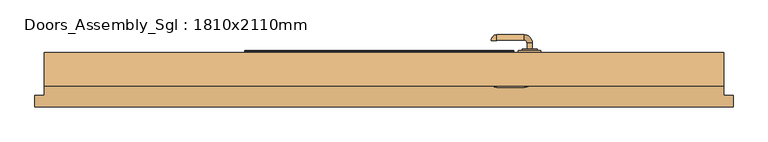
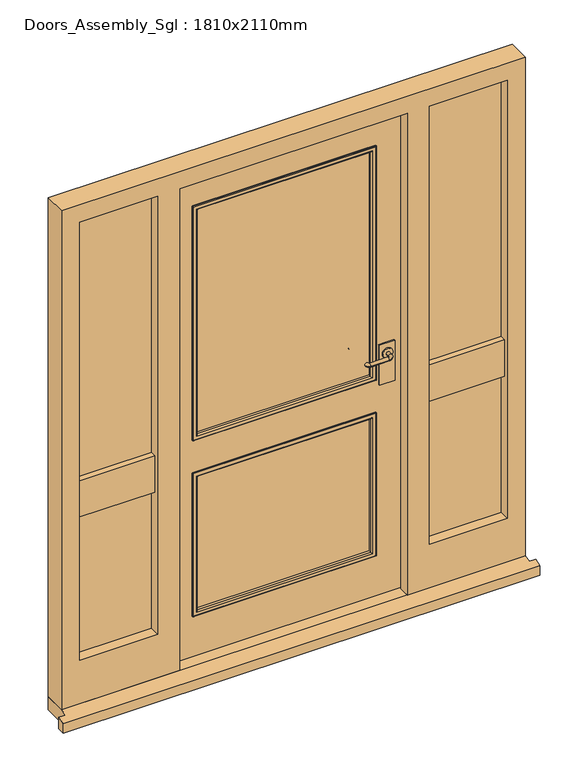
"""IFC4 building model written with IfcOpenShell, lengths in millimetres: door geometry, Doors_Assembly_Sgl : 1810x2110mm."""

from ifc_helpers import new_model, si_unit, point, frame, frame_2d, origin, place, context, project, spatial, polyline, circle_curve, ellipse_curve, trimmed, segment, composite_curve, outline, extrude, faceted_brep, source, transform, mapped, element, save
from ifc_brep_helpers import plane_surface, cylinder_surface, revolved_surface, advanced_brep


def doors_assembly_sgl_1810x2110mm_cdd653b2(model_context):
    return source(origin(), model_context, "Body", "SolidModel", [
        extrude(outline(composite_curve([segment(trimmed(circle_curve(frame_2d((1050.0, 680.0)), 20.0), [point((1050.0, 700.0))], [point((1050.0, 660.0))], False, "CARTESIAN"), True, "CONTINUOUS"), segment(trimmed(circle_curve(frame_2d((1050.0, 680.0)), 20.0), [point((1050.0, 660.0))], [point((1050.0, 700.0))], False, "CARTESIAN"), True, "CONTINUOUS")], self_intersect=False)), frame((0.0, -42.25, 0.0), z_axis=(0.0, 1.0, 0.0), x_axis=(0.0, 0.0, 1.0)), (0.0, 0.0, 1.0), 4.5929895),
        advanced_brep(
        [(673.0, -37.6570105, 1050.0), (687.0, -37.6570105, 1050.0), (687.0, -22.25, 1050.0), (673.0, -22.25, 1050.0), (665.0, -0.25, 1050.0), (665.0, -14.25, 1050.0), (593.0, -0.25, 1050.0), (593.0, -14.25, 1050.0), (592.0, -15.25, 1050.0), (578.0, -15.25, 1050.0)],
        [
            (0, 1, circle_curve(frame((680.0, -37.6570105, 1050.0), z_axis=(0.0, -1.0, 0.0), x_axis=(1.0, 0.0, 0.0)), 7.0)),
            (1, 0, circle_curve(frame((680.0, -37.6570105, 1050.0), z_axis=(0.0, -1.0, 0.0), x_axis=(1.0, 0.0, 0.0)), 7.0)),
            (1, 2),
            (2, 3, circle_curve(frame((680.0, -22.25, 1050.0), z_axis=(0.0, -1.0, 0.0), x_axis=(1.0, 0.0, 0.0)), 7.0)),
            (3, 0),
            (3, 2, circle_curve(frame((680.0, -22.25, 1050.0), z_axis=(0.0, -1.0, 0.0), x_axis=(1.0, 0.0, 0.0)), 7.0)),
            (4, 5, circle_curve(frame((665.0, -7.25, 1050.0), z_axis=(1.0, 0.0, 0.0), x_axis=(0.0, 1.0, 0.0)), 7.0)),
            (5, 3, circle_curve(frame((665.0, -22.25, 1050.0), z_axis=(0.0, 0.0, -1.0), x_axis=(1.0, 0.0, 0.0)), 8.0)),
            (2, 4, circle_curve(frame((665.0, -22.25, 1050.0), z_axis=(0.0, 0.0, 1.0), x_axis=(1.0, 0.0, 0.0)), 22.0)),
            (5, 4, circle_curve(frame((665.0, -7.25, 1050.0), z_axis=(1.0, 0.0, 0.0), x_axis=(0.0, 1.0, 0.0)), 7.0)),
            (4, 6),
            (6, 7, circle_curve(frame((593.0, -7.25, 1050.0), z_axis=(1.0, 0.0, 0.0), x_axis=(0.0, 1.0, 0.0)), 7.0)),
            (7, 5),
            (7, 6, circle_curve(frame((593.0, -7.25, 1050.0), z_axis=(1.0, 0.0, 0.0), x_axis=(0.0, 1.0, 0.0)), 7.0)),
            (8, 9, circle_curve(frame((585.0, -15.25, 1050.0), z_axis=(0.0, -1.0, 0.0), x_axis=(-1.0, 0.0, 0.0)), 7.0)),
            (9, 8, circle_curve(frame((585.0, -15.25, 1050.0), z_axis=(0.0, -1.0, 0.0), x_axis=(-1.0, 0.0, 0.0)), 7.0)),
            (8, 7, circle_curve(frame((593.0, -15.25, 1050.0), z_axis=(0.0, 0.0, -1.0), x_axis=(0.0, 1.0, 0.0)), 1.0)),
            (6, 9, circle_curve(frame((593.0, -15.25, 1050.0), z_axis=(0.0, 0.0, 1.0), x_axis=(0.0, 1.0, 0.0)), 15.0)),
        ],
        [
            plane_surface(frame((680.0, -37.6570105, 1050.0), z_axis=(0.0, -1.0, 0.0), x_axis=(0.0, 0.0, 1.0))),
            cylinder_surface(frame((680.0, -37.6570105, 1050.0), z_axis=(0.0, -1.0, 0.0), x_axis=(1.0, 0.0, 0.0)), 7.0),
            revolved_surface(trimmed(ellipse_curve(frame((680.0, -22.25, 1050.0), z_axis=(0.0, 1.0, 0.0), x_axis=(1.0, 0.0, 0.0)), 7.0, 7.0), [point((673.0, -22.25, 1050.0))], [point((687.0, -22.25, 1050.0))], True, "CARTESIAN"), (665.0, -22.25, 1050.0), (0.0, 0.0, -1.0)),
            revolved_surface(trimmed(ellipse_curve(frame((680.0, -22.25, 1050.0), z_axis=(0.0, 1.0, 0.0), x_axis=(1.0, 0.0, 0.0)), 7.0, 7.0), [point((687.0, -22.25, 1050.0))], [point((673.0, -22.25, 1050.0))], True, "CARTESIAN"), (665.0, -22.25, 1050.0), (0.0, 0.0, -1.0)),
            cylinder_surface(frame((665.0, -7.25, 1050.0), z_axis=(1.0, 0.0, 0.0), x_axis=(0.0, 1.0, 0.0)), 7.0),
            plane_surface(frame((585.0, -15.25, 1050.0), z_axis=(0.0, -1.0, 0.0), x_axis=(0.0, 0.0, 1.0))),
            revolved_surface(trimmed(ellipse_curve(frame((593.0, -7.25, 1050.0), z_axis=(-1.0, 0.0, 0.0), x_axis=(0.0, 1.0, 0.0)), 7.0, 7.0), [point((593.0, -14.25, 1050.0))], [point((593.0, -0.25, 1050.0))], True, "CARTESIAN"), (593.0, -15.25, 1050.0), (0.0, 0.0, -1.0)),
            revolved_surface(trimmed(ellipse_curve(frame((593.0, -7.25, 1050.0), z_axis=(-1.0, 0.0, 0.0), x_axis=(0.0, 1.0, 0.0)), 7.0, 7.0), [point((593.0, -0.25, 1050.0))], [point((593.0, -14.25, 1050.0))], True, "CARTESIAN"), (593.0, -15.25, 1050.0), (0.0, 0.0, -1.0)),
        ],
        [
            (0, [[1, 2]]),
            (1, [[3, 4, 5, -2]]),
            (1, [[-5, 6, -3, -1]]),
            (2, [[7, 8, -4, 9]]),
            (3, [[10, -9, -6, -8]]),
            (4, [[11, 12, 13, -7]]),
            (4, [[-13, 14, -11, -10]]),
            (5, [[15, 16]]),
            (6, [[-15, 17, -12, 18]]),
            (7, [[-16, -18, -14, -17]]),
        ],
    ),
        extrude(outline(polyline([(650.0, -48.25), (650.0, -42.25), (710.0, -42.25), (710.0, -48.25), (650.0, -48.25)])), frame((0.0, 0.0, 925.0), z_axis=(0.0, 0.0, 1.0), x_axis=(1.0, 0.0, 0.0)), (0.0, 0.0, 1.0), 165.0),
        extrude(outline(composite_curve([segment(trimmed(circle_curve(frame_2d((1050.0, 680.0)), 20.0), [point((1050.0, 700.0))], [point((1050.0, 660.0))], False, "CARTESIAN"), True, "CONTINUOUS"), segment(trimmed(circle_curve(frame_2d((1050.0, 680.0)), 20.0), [point((1050.0, 660.0))], [point((1050.0, 700.0))], False, "CARTESIAN"), True, "CONTINUOUS")], self_intersect=False)), frame((0.0, -102.8429895, 0.0), z_axis=(0.0, 1.0, 0.0), x_axis=(0.0, 0.0, 1.0)), (0.0, 0.0, 1.0), 4.5929895),
        advanced_brep(
        [(673.0, -102.8429895, 1050.0), (687.0, -102.8429895, 1050.0), (673.0, -118.25, 1050.0), (687.0, -118.25, 1050.0), (665.0, -140.25, 1050.0), (665.0, -126.25, 1050.0), (593.0, -126.25, 1050.0), (593.0, -140.25, 1050.0), (592.0, -125.25, 1050.0), (578.0, -125.25, 1050.0)],
        [
            (0, 1, circle_curve(frame((680.0, -102.8429895, 1050.0), z_axis=(0.0, 1.0, 0.0), x_axis=(1.0, 0.0, 0.0)), 7.0)),
            (1, 0, circle_curve(frame((680.0, -102.8429895, 1050.0), z_axis=(0.0, 1.0, 0.0), x_axis=(1.0, 0.0, 0.0)), 7.0)),
            (0, 2),
            (2, 3, circle_curve(frame((680.0, -118.25, 1050.0), z_axis=(0.0, 1.0, 0.0), x_axis=(1.0, 0.0, 0.0)), 7.0)),
            (3, 1),
            (3, 2, circle_curve(frame((680.0, -118.25, 1050.0), z_axis=(0.0, 1.0, 0.0), x_axis=(1.0, 0.0, 0.0)), 7.0)),
            (4, 3, circle_curve(frame((665.0, -118.25, 1050.0), z_axis=(0.0, 0.0, 1.0), x_axis=(1.0, 0.0, 0.0)), 22.0)),
            (2, 5, circle_curve(frame((665.0, -118.25, 1050.0), z_axis=(0.0, 0.0, -1.0), x_axis=(1.0, 0.0, 0.0)), 8.0)),
            (5, 4, circle_curve(frame((665.0, -133.25, 1050.0), z_axis=(1.0, 0.0, 0.0), x_axis=(0.0, -1.0, 0.0)), 7.0)),
            (4, 5, circle_curve(frame((665.0, -133.25, 1050.0), z_axis=(1.0, 0.0, 0.0), x_axis=(0.0, -1.0, 0.0)), 7.0)),
            (5, 6),
            (6, 7, circle_curve(frame((593.0, -133.25, 1050.0), z_axis=(1.0, 0.0, 0.0), x_axis=(0.0, -1.0, 0.0)), 7.0)),
            (7, 4),
            (7, 6, circle_curve(frame((593.0, -133.25, 1050.0), z_axis=(1.0, 0.0, 0.0), x_axis=(0.0, -1.0, 0.0)), 7.0)),
            (8, 9, circle_curve(frame((585.0, -125.25, 1050.0), z_axis=(0.0, 1.0, 0.0), x_axis=(-1.0, 0.0, 0.0)), 7.0)),
            (9, 8, circle_curve(frame((585.0, -125.25, 1050.0), z_axis=(0.0, 1.0, 0.0), x_axis=(-1.0, 0.0, 0.0)), 7.0)),
            (9, 7, circle_curve(frame((593.0, -125.25, 1050.0), z_axis=(0.0, 0.0, 1.0), x_axis=(0.0, -1.0, 0.0)), 15.0)),
            (6, 8, circle_curve(frame((593.0, -125.25, 1050.0), z_axis=(0.0, 0.0, -1.0), x_axis=(0.0, -1.0, 0.0)), 1.0)),
        ],
        [
            plane_surface(frame((680.0, -102.8429895, 1050.0), z_axis=(0.0, 1.0, 0.0), x_axis=(0.0, 0.0, 1.0))),
            cylinder_surface(frame((680.0, -102.8429895, 1050.0), z_axis=(0.0, 1.0, 0.0), x_axis=(1.0, 0.0, 0.0)), 7.0),
            revolved_surface(trimmed(ellipse_curve(frame((680.0, -118.25, 1050.0), z_axis=(0.0, 1.0, 0.0), x_axis=(1.0, 0.0, 0.0)), 7.0, 7.0), [point((673.0, -118.25, 1050.0))], [point((687.0, -118.25, 1050.0))], True, "CARTESIAN"), (665.0, -118.25, 1050.0), (0.0, 0.0, -1.0)),
            revolved_surface(trimmed(ellipse_curve(frame((680.0, -118.25, 1050.0), z_axis=(0.0, 1.0, 0.0), x_axis=(1.0, 0.0, 0.0)), 7.0, 7.0), [point((687.0, -118.25, 1050.0))], [point((673.0, -118.25, 1050.0))], True, "CARTESIAN"), (665.0, -118.25, 1050.0), (0.0, 0.0, -1.0)),
            cylinder_surface(frame((665.0, -133.25, 1050.0), z_axis=(1.0, 0.0, 0.0), x_axis=(0.0, -1.0, 0.0)), 7.0),
            plane_surface(frame((585.0, -125.25, 1050.0), z_axis=(0.0, 1.0, 0.0), x_axis=(0.0, 0.0, 1.0))),
            revolved_surface(trimmed(ellipse_curve(frame((593.0, -133.25, 1050.0), z_axis=(1.0, 0.0, 0.0), x_axis=(0.0, -1.0, 0.0)), 7.0, 7.0), [point((593.0, -126.25, 1050.0))], [point((593.0, -140.25, 1050.0))], True, "CARTESIAN"), (593.0, -125.25, 1050.0), (0.0, 0.0, -1.0)),
            revolved_surface(trimmed(ellipse_curve(frame((593.0, -133.25, 1050.0), z_axis=(1.0, 0.0, 0.0), x_axis=(0.0, -1.0, 0.0)), 7.0, 7.0), [point((593.0, -140.25, 1050.0))], [point((593.0, -126.25, 1050.0))], True, "CARTESIAN"), (593.0, -125.25, 1050.0), (0.0, 0.0, -1.0)),
        ],
        [
            (0, [[1, 2]]),
            (1, [[-1, 3, 4, 5]]),
            (1, [[-2, -5, 6, -3]]),
            (2, [[7, -4, 8, 9]]),
            (3, [[-8, -6, -7, 10]]),
            (4, [[-9, 11, 12, 13]]),
            (4, [[-10, -13, 14, -11]]),
            (5, [[15, 16]]),
            (6, [[17, -12, 18, -16]]),
            (7, [[-18, -14, -17, -15]]),
        ],
    ),
        extrude(outline(polyline([(650.0, -92.25), (710.0, -92.25), (710.0, -98.25), (650.0, -98.25), (650.0, -92.25)])), frame((0.0, 0.0, 925.0), z_axis=(0.0, 0.0, 1.0), x_axis=(1.0, 0.0, 0.0)), (0.0, 0.0, 1.0), 165.0),
        extrude(outline(polyline([(1148.5, -71.25), (1148.5, -95.25), (800.0, -95.25), (800.0, -71.25), (1148.5, -71.25)])), frame((0.0, 0.0, 218.5), z_axis=(0.0, 0.0, 1.0), x_axis=(1.0, 0.0, 0.0)), (0.0, 0.0, 1.0), 605.0),
        extrude(outline(polyline([(1148.5, -71.25), (1148.5, -95.25), (800.0, -95.25), (800.0, -71.25), (1148.5, -71.25)])), frame((0.0, 0.0, 943.5), z_axis=(0.0, 0.0, 1.0), x_axis=(1.0, 0.0, 0.0)), (0.0, 0.0, 1.0), 1118.0),
        extrude(outline(polyline([(-216.0, -71.25), (-216.0, -95.25), (-564.5, -95.25), (-564.5, -71.25), (-216.0, -71.25)])), frame((0.0, 0.0, 218.5), z_axis=(0.0, 0.0, 1.0), x_axis=(1.0, 0.0, 0.0)), (0.0, 0.0, 1.0), 605.0),
        extrude(outline(polyline([(-216.0, -71.25), (-216.0, -95.25), (-564.5, -95.25), (-564.5, -71.25), (-216.0, -71.25)])), frame((0.0, 0.0, 943.5), z_axis=(0.0, 0.0, 1.0), x_axis=(1.0, 0.0, 0.0)), (0.0, 0.0, 1.0), 1118.0),
        faceted_brep([(1197.0, -137.25, 54.5), (736.0, -137.25, 54.5), (736.0, -95.25, 54.5), (758.0, -95.25, 54.5), (758.0, -48.25, 54.5), (1197.0, -48.25, 54.5), (1197.0, -48.25, 2110.0), (1197.0, -137.25, 2110.0), (758.0, -48.25, 2061.5), (-174.0, -48.25, 2061.5), (-174.0, -48.25, 54.5), (-613.0, -48.25, 54.5), (-613.0, -48.25, 2110.0), (1126.5, -48.25, 958.5), (1126.5, -48.25, 2039.5), (822.0, -48.25, 2039.5), (822.0, -48.25, 958.5), (822.0, -48.25, 808.5), (822.0, -48.25, 233.5), (1126.5, -48.25, 233.5), (1126.5, -48.25, 808.5), (-238.0, -48.25, 808.5), (-542.5, -48.25, 808.5), (-542.5, -48.25, 233.5), (-238.0, -48.25, 233.5), (-542.5, -48.25, 2039.5), (-542.5, -48.25, 958.5), (-238.0, -48.25, 958.5), (-238.0, -48.25, 2039.5), (758.0, -95.25, 2061.5), (-174.0, -95.25, 54.5), (-174.0, -95.25, 2061.5), (736.0, -95.25, 2039.5), (-152.0, -95.25, 2039.5), (-152.0, -95.25, 54.5), (-216.0, -95.25, 2061.5), (-216.0, -95.25, 943.5), (-564.5, -95.25, 943.5), (-564.5, -95.25, 2061.5), (-542.5, -95.25, 2039.5), (-542.5, -95.25, 958.5), (-238.0, -95.25, 958.5), (-238.0, -95.25, 2039.5), (1148.5, -95.25, 2061.5), (1148.5, -95.25, 943.5), (800.0, -95.25, 943.5), (800.0, -95.25, 2061.5), (822.0, -95.25, 2039.5), (822.0, -95.25, 958.5), (1126.5, -95.25, 958.5), (1126.5, -95.25, 2039.5), (1148.5, -95.25, 218.5), (800.0, -95.25, 218.5), (800.0, -95.25, 823.5), (1148.5, -95.25, 823.5), (1126.5, -95.25, 808.5), (822.0, -95.25, 808.5), (822.0, -95.25, 233.5), (1126.5, -95.25, 233.5), (-564.5, -95.25, 823.5), (-216.0, -95.25, 823.5), (-216.0, -95.25, 218.5), (-564.5, -95.25, 218.5), (-238.0, -95.25, 808.5), (-542.5, -95.25, 808.5), (-542.5, -95.25, 233.5), (-238.0, -95.25, 233.5), (736.0, -137.25, 2039.5), (-613.0, -137.25, 54.5), (-152.0, -137.25, 54.5), (-152.0, -137.25, 2039.5), (-613.0, -137.25, 2110.0), (-238.0, -137.25, 2039.5), (-238.0, -137.25, 233.5), (-542.5, -137.25, 233.5), (-542.5, -137.25, 2039.5), (1126.5, -137.25, 2039.5), (1126.5, -137.25, 233.5), (822.0, -137.25, 233.5), (822.0, -137.25, 2039.5), (-542.5, -118.25, 808.5), (-542.5, -118.25, 958.5), (-238.0, -118.25, 958.5), (-238.0, -118.25, 808.5), (822.0, -118.25, 808.5), (822.0, -118.25, 958.5), (1126.5, -118.25, 958.5), (1126.5, -118.25, 808.5), (822.0, -71.25, 958.5), (1126.5, -71.25, 958.5), (822.0, -71.25, 2039.5), (822.0, -71.25, 808.5), (822.0, -71.25, 233.5), (1126.5, -71.25, 2039.5), (1126.5, -71.25, 233.5), (1126.5, -71.25, 808.5), (-238.0, -71.25, 958.5), (-238.0, -71.25, 2039.5), (-238.0, -71.25, 233.5), (-238.0, -71.25, 808.5), (-542.5, -71.25, 233.5), (-542.5, -71.25, 2039.5), (-542.5, -71.25, 958.5), (-542.5, -71.25, 808.5), (1148.5, -71.25, 218.5), (1148.5, -71.25, 823.5), (1148.5, -71.25, 943.5), (1148.5, -71.25, 2061.5), (800.0, -71.25, 823.5), (800.0, -71.25, 218.5), (800.0, -71.25, 2061.5), (800.0, -71.25, 943.5), (-564.5, -71.25, 218.5), (-564.5, -71.25, 823.5), (-564.5, -71.25, 943.5), (-564.5, -71.25, 2061.5), (-216.0, -71.25, 943.5), (-216.0, -71.25, 2061.5), (-216.0, -71.25, 823.5), (-216.0, -71.25, 218.5)], [[[0, 1, 2, 3, 4, 5]], [[5, 6, 7, 0]], [[5, 4, 8, 9, 10, 11, 12, 6], [13, 14, 15, 16], [17, 18, 19, 20], [21, 22, 23, 24], [25, 26, 27, 28]], [[3, 29, 8, 4]], [[30, 31, 29, 3, 2, 32, 33, 34]], [[35, 36, 37, 38], [39, 40, 41, 42]], [[43, 44, 45, 46], [47, 48, 49, 50]], [[51, 52, 53, 54], [55, 56, 57, 58]], [[59, 60, 61, 62], [63, 64, 65, 66]], [[1, 67, 32, 2]], [[68, 69, 70, 67, 1, 0, 7, 71], [72, 73, 74, 75], [76, 77, 78, 79]], [[71, 12, 11, 68]], [[34, 33, 70, 69]], [[11, 10, 30, 34, 69, 68]], [[75, 74, 65, 64, 80, 81, 40, 39]], [[65, 74, 73, 66]], [[42, 41, 82, 83, 63, 66, 73, 72]], [[79, 78, 57, 56, 84, 85, 48, 47]], [[77, 58, 57, 78]], [[50, 49, 86, 87, 55, 58, 77, 76]], [[16, 88, 89, 13]], [[90, 88, 16, 15]], [[17, 91, 92, 18]], [[14, 13, 89, 93]], [[19, 94, 95, 20]], [[20, 95, 91, 17]], [[18, 92, 94, 19]], [[28, 27, 96, 97]], [[24, 98, 99, 21]], [[23, 100, 98, 24]], [[101, 102, 26, 25]], [[22, 103, 100, 23]], [[21, 99, 103, 22]], [[26, 102, 96, 27]], [[10, 9, 31, 30]], [[104, 51, 54, 105]], [[106, 44, 43, 107]], [[104, 105, 108, 109], [94, 92, 91, 95]], [[110, 111, 106, 107], [93, 89, 88, 90]], [[54, 53, 108, 105]], [[109, 52, 51, 104]], [[111, 45, 44, 106]], [[40, 81, 82, 41]], [[112, 113, 59, 62]], [[114, 115, 38, 37]], [[37, 36, 116, 114]], [[36, 35, 117, 116]], [[61, 60, 118, 119]], [[48, 85, 86, 49]], [[108, 53, 52, 109]], [[110, 46, 45, 111]], [[55, 87, 84, 56]], [[63, 83, 80, 64]], [[112, 62, 61, 119]], [[113, 118, 60, 59]], [[85, 84, 87, 86]], [[115, 114, 116, 117], [97, 96, 102, 101]], [[119, 118, 113, 112], [100, 103, 99, 98]], [[81, 80, 83, 82]], [[7, 6, 12, 71]], [[9, 8, 29, 31]], [[38, 115, 117, 35]], [[46, 110, 107, 43]], [[76, 79, 47, 50]], [[33, 32, 67, 70]], [[39, 42, 72, 75]], [[101, 25, 28, 97]], [[14, 93, 90, 15]]]),
        extrude(outline(polyline([(-71.0, -82.25), (-71.0, -58.25), (630.0, -58.25), (630.0, -82.25), (-71.0, -82.25)])), frame((0.0, 0.0, 958.5), z_axis=(0.0, 0.0, 1.0), x_axis=(1.0, 0.0, 0.0)), (0.0, 0.0, 1.0), 950.0),
        extrude(outline(polyline([(-71.0, -82.25), (-71.0, -58.25), (630.0, -58.25), (630.0, -82.25), (-71.0, -82.25)])), frame((0.0, 0.0, 233.5), z_axis=(0.0, 0.0, 1.0), x_axis=(1.0, 0.0, 0.0)), (0.0, 0.0, 1.0), 575.0),
        faceted_brep([(1222.0, -192.25, 0.0), (1222.0, -162.25, 0.0), (1222.0, -162.25, 47.2703282), (1222.0, -192.25, 38.5947221), (-638.0, -192.25, 38.5947221), (-638.0, -162.25, 47.2703282), (-638.0, -162.25, 0.0), (-638.0, -192.25, 0.0), (-613.0, -162.25, 0.0), (-613.0, -48.25, 0.0), (1197.0, -48.25, 0.0), (1197.0, -162.25, 0.0), (1197.0, -162.25, 47.2703282), (1197.0, -137.25, 54.5), (-613.0, -137.25, 54.5), (-613.0, -162.25, 47.2703282), (1197.0, -48.25, 54.5), (-613.0, -48.25, 54.5)], [[[0, 1, 2, 3]], [[4, 5, 6, 7]], [[7, 6, 8, 9, 10, 11, 1, 0]], [[3, 4, 7, 0]], [[3, 2, 12, 13, 14, 15, 5, 4]], [[14, 13, 16, 17]], [[17, 16, 10, 9]], [[15, 14, 17, 9, 8]], [[8, 6, 5, 15]], [[11, 10, 16, 13, 12]], [[12, 2, 1, 11]]]),
        extrude(outline(polyline([(58.5, -171.0), (58.5, 755.0), (2058.5, 755.0), (2058.5, -171.0), (58.5, -171.0)]), holes=[polyline([(1908.5, 630.0), (958.5, 630.0), (958.5, -71.0), (1908.5, -71.0), (1908.5, 630.0)]), polyline([(808.5, -71.0), (808.5, 630.0), (233.5, 630.0), (233.5, -71.0), (808.5, -71.0)])]), frame((0.0, -92.25, 0.0), z_axis=(0.0, 1.0, 0.0), x_axis=(0.0, 0.0, 1.0)), (0.0, 0.0, 1.0), 44.0),
        advanced_brep(
        [(630.0, -58.25, 808.5), (630.0, -58.25, 233.5), (630.0, -48.25, 233.5), (630.0, -48.25, 808.5), (618.0, -47.25, 796.5), (618.0, -47.25, 245.5), (618.0, -58.25, 245.5), (618.0, -58.25, 796.5), (623.0, -42.25, 801.5), (623.0, -42.25, 240.5), (638.0, -44.25, 816.5), (638.0, -44.25, 225.5), (636.0, -42.25, 227.5), (636.0, -42.25, 814.5), (638.0, -48.25, 816.5), (638.0, -48.25, 225.5), (-71.0, -58.25, 233.5), (-71.0, -48.25, 233.5), (-59.0, -47.25, 245.5), (-59.0, -58.25, 245.5), (-64.0, -42.25, 240.5), (-79.0, -44.25, 225.5), (-77.0, -42.25, 227.5), (-79.0, -48.25, 225.5), (-71.0, -58.25, 808.5), (-71.0, -48.25, 808.5), (-59.0, -47.25, 796.5), (-59.0, -58.25, 796.5), (-64.0, -42.25, 801.5), (-79.0, -44.25, 816.5), (-77.0, -42.25, 814.5), (-79.0, -48.25, 816.5)],
        [
            (0, 1),
            (1, 2),
            (2, 3),
            (3, 0),
            (4, 5),
            (5, 6),
            (6, 7),
            (7, 4),
            (8, 9),
            (9, 5, ellipse_curve(frame((623.0, -47.25, 240.5), z_axis=(0.7071067811865429, 0.0, 0.707106781186552), x_axis=(-0.7071067811865519, 0.0, 0.7071067811865431)), 7.0710678, 5.0)),
            (4, 8, ellipse_curve(frame((623.0, -47.25, 801.5), z_axis=(0.707106781186552, 0.0, -0.707106781186543), x_axis=(0.7071067811865429, 0.0, 0.707106781186552)), 7.0710678, 5.0)),
            (10, 11),
            (11, 12, ellipse_curve(frame((636.0, -44.25, 227.5), z_axis=(0.7071067811865429, 0.0, 0.707106781186552), x_axis=(-0.7071067811865519, 0.0, 0.7071067811865431)), 2.8284271, 2.0)),
            (12, 13),
            (13, 10, ellipse_curve(frame((636.0, -44.25, 814.5), z_axis=(0.707106781186552, 0.0, -0.707106781186543), x_axis=(0.7071067811865429, 0.0, 0.707106781186552)), 2.8284271, 2.0)),
            (14, 15),
            (15, 11),
            (10, 14),
            (1, 16),
            (16, 17),
            (17, 2),
            (5, 18),
            (18, 19),
            (19, 6),
            (9, 20),
            (20, 18, ellipse_curve(frame((-64.0, -47.25, 240.5), z_axis=(0.707106781186552, 0.0, -0.7071067811865431), x_axis=(0.7071067811865429, 0.0, 0.707106781186552)), 7.0710678, 5.0)),
            (11, 21),
            (21, 22, ellipse_curve(frame((-77.0, -44.25, 227.5), z_axis=(0.707106781186552, 0.0, -0.7071067811865431), x_axis=(0.7071067811865429, 0.0, 0.707106781186552)), 2.8284271, 2.0)),
            (22, 12),
            (15, 23),
            (23, 21),
            (16, 24),
            (24, 25),
            (25, 17),
            (18, 26),
            (26, 27),
            (27, 19),
            (20, 28),
            (28, 26, ellipse_curve(frame((-64.0, -47.25, 801.5), z_axis=(-0.707106781186543, 0.0, -0.7071067811865519), x_axis=(0.7071067811865518, 0.0, -0.7071067811865431)), 7.0710678, 5.0)),
            (21, 29),
            (29, 30, ellipse_curve(frame((-77.0, -44.25, 814.5), z_axis=(-0.707106781186543, 0.0, -0.7071067811865519), x_axis=(0.7071067811865518, 0.0, -0.7071067811865431)), 2.8284271, 2.0)),
            (30, 22),
            (23, 31),
            (31, 29),
            (14, 31),
            (25, 3),
            (24, 0),
            (27, 7),
            (26, 4),
            (28, 8),
            (30, 13),
            (29, 10),
        ],
        [
            plane_surface(frame((630.0, -48.25, 808.5), z_axis=(1.0, 0.0, 0.0), x_axis=(0.0, 0.0, -1.0))),
            plane_surface(frame((618.0, -58.25, 796.5), z_axis=(-1.0, 0.0, 0.0), x_axis=(0.0, 0.0, -1.0))),
            cylinder_surface(frame((623.0, -47.25, 808.5), z_axis=(0.0, 0.0, 1.0), x_axis=(1.0, 0.0, 0.0)), 5.0),
            cylinder_surface(frame((636.0, -44.25, 808.5), z_axis=(0.0, 0.0, 1.0), x_axis=(1.0, 0.0, 0.0)), 2.0),
            plane_surface(frame((638.0, -44.25, 816.5), z_axis=(1.0, 0.0, 0.0), x_axis=(0.0, 0.0, -1.0))),
            plane_surface(frame((630.0, -48.25, 233.5), z_axis=(0.0, 0.0, -1.0), x_axis=(-1.0, 0.0, 0.0))),
            plane_surface(frame((618.0, -58.25, 245.5), z_axis=(0.0, 0.0, 1.0), x_axis=(-1.0, 0.0, 0.0))),
            cylinder_surface(frame((630.0, -47.25, 240.5), z_axis=(1.0, 0.0, 0.0), x_axis=(0.0, 0.0, -1.0)), 5.0),
            cylinder_surface(frame((630.0, -44.25, 227.5), z_axis=(1.0, 0.0, 0.0), x_axis=(0.0, 0.0, -1.0)), 2.0),
            plane_surface(frame((638.0, -44.25, 225.5), z_axis=(0.0, 0.0, -1.0), x_axis=(-1.0, 0.0, 0.0))),
            plane_surface(frame((-71.0, -48.25, 233.5), z_axis=(-1.0, 0.0, 0.0), x_axis=(0.0, 0.0, 1.0))),
            plane_surface(frame((-59.0, -58.25, 245.5), z_axis=(1.0, 0.0, 0.0), x_axis=(0.0, 0.0, 1.0))),
            cylinder_surface(frame((-64.0, -47.25, 233.5), z_axis=(0.0, 0.0, -1.0), x_axis=(-1.0, 0.0, 0.0)), 5.0),
            cylinder_surface(frame((-77.0, -44.25, 233.5), z_axis=(0.0, 0.0, -1.0), x_axis=(-1.0, 0.0, 0.0)), 2.0),
            plane_surface(frame((-79.0, -44.25, 225.5), z_axis=(-1.0, 0.0, 0.0), x_axis=(0.0, 0.0, 1.0))),
            plane_surface(frame((-79.0, -48.25, 816.5), z_axis=(0.0, -1.0, 0.0), x_axis=(1.0, 0.0, 0.0))),
            plane_surface(frame((-71.0, -48.25, 808.5), z_axis=(0.0, 0.0, 1.0), x_axis=(1.0, 0.0, 0.0))),
            plane_surface(frame((-71.0, -58.25, 808.5), z_axis=(0.0, -1.0, 0.0), x_axis=(1.0, 0.0, 0.0))),
            plane_surface(frame((-59.0, -58.25, 796.5), z_axis=(0.0, 0.0, -1.0), x_axis=(1.0, 0.0, 0.0))),
            cylinder_surface(frame((-71.0, -47.25, 801.5), z_axis=(-1.0, 0.0, 0.0), x_axis=(0.0, 0.0, 1.0)), 5.0),
            plane_surface(frame((-64.0, -42.25, 801.5), z_axis=(0.0, 1.0, 0.0), x_axis=(1.0, 0.0, 0.0))),
            cylinder_surface(frame((-71.0, -44.25, 814.5), z_axis=(-1.0, 0.0, 0.0), x_axis=(0.0, 0.0, 1.0)), 2.0),
            plane_surface(frame((-79.0, -44.25, 816.5), z_axis=(0.0, 0.0, 1.0), x_axis=(1.0, 0.0, 0.0))),
        ],
        [
            (0, [[1, 2, 3, 4]]),
            (1, [[5, 6, 7, 8]]),
            (2, [[9, 10, -5, 11]]),
            (3, [[12, 13, 14, 15]]),
            (4, [[16, 17, -12, 18]]),
            (5, [[19, 20, 21, -2]]),
            (6, [[22, 23, 24, -6]]),
            (7, [[25, 26, -22, -10]]),
            (8, [[27, 28, 29, -13]]),
            (9, [[30, 31, -27, -17]]),
            (10, [[32, 33, 34, -20]]),
            (11, [[35, 36, 37, -23]]),
            (12, [[38, 39, -35, -26]]),
            (13, [[40, 41, 42, -28]]),
            (14, [[43, 44, -40, -31]]),
            (15, [[-16, 45, -43, -30], [-3, -21, -34, 46]]),
            (16, [[47, -4, -46, -33]]),
            (17, [[-1, -47, -32, -19], [-7, -24, -37, 48]]),
            (18, [[49, -8, -48, -36]]),
            (19, [[50, -11, -49, -39]]),
            (20, [[-14, -29, -42, 51], [-9, -50, -38, -25]]),
            (21, [[52, -15, -51, -41]]),
            (22, [[-45, -18, -52, -44]]),
        ],
    ),
        advanced_brep(
        [(-71.0, -82.25, 808.5), (-71.0, -82.25, 233.5), (-71.0, -92.25, 233.5), (-71.0, -92.25, 808.5), (-59.0, -93.25, 796.5), (-59.0, -93.25, 245.5), (-59.0, -82.25, 245.5), (-59.0, -82.25, 796.5), (-64.0, -98.25, 801.5), (-64.0, -98.25, 240.5), (-79.0, -96.25, 816.5), (-79.0, -96.25, 225.5), (-77.0, -98.25, 227.5), (-77.0, -98.25, 814.5), (-79.0, -92.25, 816.5), (-79.0, -92.25, 225.5), (630.0, -82.25, 233.5), (630.0, -92.25, 233.5), (618.0, -93.25, 245.5), (618.0, -82.25, 245.5), (623.0, -98.25, 240.5), (638.0, -96.25, 225.5), (636.0, -98.25, 227.5), (638.0, -92.25, 225.5), (630.0, -82.25, 808.5), (630.0, -92.25, 808.5), (618.0, -93.25, 796.5), (618.0, -82.25, 796.5), (623.0, -98.25, 801.5), (638.0, -96.25, 816.5), (636.0, -98.25, 814.5), (638.0, -92.25, 816.5)],
        [
            (0, 1),
            (1, 2),
            (2, 3),
            (3, 0),
            (4, 5),
            (5, 6),
            (6, 7),
            (7, 4),
            (8, 9),
            (9, 5, ellipse_curve(frame((-64.0, -93.25, 240.5), z_axis=(-0.7071067811865475, 0.0, 0.7071067811865475), x_axis=(0.7071067811865474, 0.0, 0.7071067811865476)), 7.0710678, 5.0)),
            (4, 8, ellipse_curve(frame((-64.0, -93.25, 801.5), z_axis=(-0.7071067811865475, 0.0, -0.7071067811865475), x_axis=(-0.7071067811865474, 0.0, 0.7071067811865477)), 7.0710678, 5.0)),
            (10, 11),
            (11, 12, ellipse_curve(frame((-77.0, -96.25, 227.5), z_axis=(-0.7071067811865475, 0.0, 0.7071067811865475), x_axis=(0.7071067811865474, 0.0, 0.7071067811865476)), 2.8284271, 2.0)),
            (12, 13),
            (13, 10, ellipse_curve(frame((-77.0, -96.25, 814.5), z_axis=(-0.7071067811865475, 0.0, -0.7071067811865475), x_axis=(-0.7071067811865474, 0.0, 0.7071067811865477)), 2.8284271, 2.0)),
            (14, 15),
            (15, 11),
            (10, 14),
            (1, 16),
            (16, 17),
            (17, 2),
            (5, 18),
            (18, 19),
            (19, 6),
            (9, 20),
            (20, 18, ellipse_curve(frame((623.0, -93.25, 240.5), z_axis=(-0.7071067811865475, 0.0, -0.7071067811865475), x_axis=(-0.7071067811865476, 0.0, 0.7071067811865474)), 7.0710678, 5.0)),
            (11, 21),
            (21, 22, ellipse_curve(frame((636.0, -96.25, 227.5), z_axis=(-0.7071067811865475, 0.0, -0.7071067811865475), x_axis=(-0.7071067811865476, 0.0, 0.7071067811865474)), 2.8284271, 2.0)),
            (22, 12),
            (15, 23),
            (23, 21),
            (16, 24),
            (24, 25),
            (25, 17),
            (18, 26),
            (26, 27),
            (27, 19),
            (20, 28),
            (28, 26, ellipse_curve(frame((623.0, -93.25, 801.5), z_axis=(0.7071067811865475, 0.0, -0.7071067811865475), x_axis=(-0.7071067811865474, 0.0, -0.7071067811865477)), 7.0710678, 5.0)),
            (21, 29),
            (29, 30, ellipse_curve(frame((636.0, -96.25, 814.5), z_axis=(0.7071067811865475, 0.0, -0.7071067811865475), x_axis=(-0.7071067811865474, 0.0, -0.7071067811865477)), 2.8284271, 2.0)),
            (30, 22),
            (23, 31),
            (31, 29),
            (14, 31),
            (25, 3),
            (24, 0),
            (27, 7),
            (26, 4),
            (28, 8),
            (30, 13),
            (29, 10),
        ],
        [
            plane_surface(frame((-71.0, -92.25, 808.5), z_axis=(-1.0, 0.0, 0.0), x_axis=(0.0, 0.0, -1.0))),
            plane_surface(frame((-59.0, -82.25, 796.5), z_axis=(1.0, 0.0, 0.0), x_axis=(0.0, 0.0, -1.0))),
            cylinder_surface(frame((-64.0, -93.25, 808.5), z_axis=(0.0, 0.0, 1.0), x_axis=(-1.0, 0.0, 0.0)), 5.0),
            cylinder_surface(frame((-77.0, -96.25, 808.5), z_axis=(0.0, 0.0, 1.0), x_axis=(-1.0, 0.0, 0.0)), 2.0),
            plane_surface(frame((-79.0, -96.25, 816.5), z_axis=(-1.0, 0.0, 0.0), x_axis=(0.0, 0.0, -1.0))),
            plane_surface(frame((-71.0, -92.25, 233.5), z_axis=(0.0, 0.0, -1.0), x_axis=(1.0, 0.0, 0.0))),
            plane_surface(frame((-59.0, -82.25, 245.5), z_axis=(0.0, 0.0, 1.0), x_axis=(1.0, 0.0, 0.0))),
            cylinder_surface(frame((-71.0, -93.25, 240.5), z_axis=(-1.0, 0.0, 0.0), x_axis=(0.0, 0.0, -1.0)), 5.0),
            cylinder_surface(frame((-71.0, -96.25, 227.5), z_axis=(-1.0, 0.0, 0.0), x_axis=(0.0, 0.0, -1.0)), 2.0),
            plane_surface(frame((-79.0, -96.25, 225.5), z_axis=(0.0, 0.0, -1.0), x_axis=(1.0, 0.0, 0.0))),
            plane_surface(frame((630.0, -92.25, 233.5), z_axis=(1.0, 0.0, 0.0), x_axis=(0.0, 0.0, 1.0))),
            plane_surface(frame((618.0, -82.25, 245.5), z_axis=(-1.0, 0.0, 0.0), x_axis=(0.0, 0.0, 1.0))),
            cylinder_surface(frame((623.0, -93.25, 233.5), z_axis=(0.0, 0.0, -1.0), x_axis=(1.0, 0.0, 0.0)), 5.0),
            cylinder_surface(frame((636.0, -96.25, 233.5), z_axis=(0.0, 0.0, -1.0), x_axis=(1.0, 0.0, 0.0)), 2.0),
            plane_surface(frame((638.0, -96.25, 225.5), z_axis=(1.0, 0.0, 0.0), x_axis=(0.0, 0.0, 1.0))),
            plane_surface(frame((638.0, -92.25, 816.5), z_axis=(0.0, 1.0, 0.0), x_axis=(-1.0, 0.0, 0.0))),
            plane_surface(frame((630.0, -92.25, 808.5), z_axis=(0.0, 0.0, 1.0), x_axis=(-1.0, 0.0, 0.0))),
            plane_surface(frame((630.0, -82.25, 808.5), z_axis=(0.0, 1.0, 0.0), x_axis=(-1.0, 0.0, 0.0))),
            plane_surface(frame((618.0, -82.25, 796.5), z_axis=(0.0, 0.0, -1.0), x_axis=(-1.0, 0.0, 0.0))),
            cylinder_surface(frame((630.0, -93.25, 801.5), z_axis=(1.0, 0.0, 0.0), x_axis=(0.0, 0.0, 1.0)), 5.0),
            plane_surface(frame((623.0, -98.25, 801.5), z_axis=(0.0, -1.0, 0.0), x_axis=(-1.0, 0.0, 0.0))),
            cylinder_surface(frame((630.0, -96.25, 814.5), z_axis=(1.0, 0.0, 0.0), x_axis=(0.0, 0.0, 1.0)), 2.0),
            plane_surface(frame((638.0, -96.25, 816.5), z_axis=(0.0, 0.0, 1.0), x_axis=(-1.0, 0.0, 0.0))),
        ],
        [
            (0, [[1, 2, 3, 4]]),
            (1, [[5, 6, 7, 8]]),
            (2, [[9, 10, -5, 11]]),
            (3, [[12, 13, 14, 15]]),
            (4, [[16, 17, -12, 18]]),
            (5, [[19, 20, 21, -2]]),
            (6, [[22, 23, 24, -6]]),
            (7, [[25, 26, -22, -10]]),
            (8, [[27, 28, 29, -13]]),
            (9, [[30, 31, -27, -17]]),
            (10, [[32, 33, 34, -20]]),
            (11, [[35, 36, 37, -23]]),
            (12, [[38, 39, -35, -26]]),
            (13, [[40, 41, 42, -28]]),
            (14, [[43, 44, -40, -31]]),
            (15, [[-16, 45, -43, -30], [-3, -21, -34, 46]]),
            (16, [[47, -4, -46, -33]]),
            (17, [[-1, -47, -32, -19], [-7, -24, -37, 48]]),
            (18, [[49, -8, -48, -36]]),
            (19, [[50, -11, -49, -39]]),
            (20, [[-14, -29, -42, 51], [-9, -50, -38, -25]]),
            (21, [[52, -15, -51, -41]]),
            (22, [[-45, -18, -52, -44]]),
        ],
    ),
        advanced_brep(
        [(-79.0, -96.25, 950.5), (-79.0, -96.25, 1916.5), (-79.0, -92.25, 1916.5), (-79.0, -92.25, 950.5), (-77.0, -98.25, 952.5), (-77.0, -98.25, 1914.5), (-59.0, -93.25, 970.5), (-59.0, -93.25, 1896.5), (-64.0, -98.25, 1901.5), (-64.0, -98.25, 965.5), (-59.0, -82.25, 970.5), (-59.0, -82.25, 1896.5), (-71.0, -92.25, 958.5), (-71.0, -92.25, 1908.5), (-71.0, -82.25, 1908.5), (-71.0, -82.25, 958.5), (638.0, -96.25, 1916.5), (638.0, -92.25, 1916.5), (636.0, -98.25, 1914.5), (618.0, -93.25, 1896.5), (623.0, -98.25, 1901.5), (618.0, -82.25, 1896.5), (630.0, -92.25, 1908.5), (630.0, -82.25, 1908.5), (638.0, -96.25, 950.5), (638.0, -92.25, 950.5), (636.0, -98.25, 952.5), (618.0, -93.25, 970.5), (623.0, -98.25, 965.5), (618.0, -82.25, 970.5), (630.0, -92.25, 958.5), (630.0, -82.25, 958.5)],
        [
            (0, 1),
            (1, 2),
            (2, 3),
            (3, 0),
            (4, 5),
            (5, 1, ellipse_curve(frame((-77.0, -96.25, 1914.5), z_axis=(-0.7071067811865476, 0.0, -0.7071067811865474), x_axis=(0.7071067811865472, 0.0, -0.7071067811865478)), 2.8284271, 2.0)),
            (0, 4, ellipse_curve(frame((-77.0, -96.25, 952.5), z_axis=(-0.7071067811865474, 0.0, 0.7071067811865476), x_axis=(-0.7071067811865475, 0.0, -0.7071067811865475)), 2.8284271, 2.0)),
            (6, 7),
            (7, 8, ellipse_curve(frame((-64.0, -93.25, 1901.5), z_axis=(-0.7071067811865476, 0.0, -0.7071067811865474), x_axis=(0.7071067811865472, 0.0, -0.7071067811865478)), 7.0710678, 5.0)),
            (8, 9),
            (9, 6, ellipse_curve(frame((-64.0, -93.25, 965.5), z_axis=(-0.7071067811865474, 0.0, 0.7071067811865476), x_axis=(-0.7071067811865475, 0.0, -0.7071067811865475)), 7.0710678, 5.0)),
            (10, 11),
            (11, 7),
            (6, 10),
            (12, 13),
            (13, 14),
            (14, 15),
            (15, 12),
            (1, 16),
            (16, 17),
            (17, 2),
            (5, 18),
            (18, 16, ellipse_curve(frame((636.0, -96.25, 1914.5), z_axis=(-0.7071067811865474, 0.0, 0.7071067811865476), x_axis=(-0.7071067811865477, 0.0, -0.7071067811865472)), 2.8284271, 2.0)),
            (7, 19),
            (19, 20, ellipse_curve(frame((623.0, -93.25, 1901.5), z_axis=(-0.7071067811865474, 0.0, 0.7071067811865476), x_axis=(-0.7071067811865477, 0.0, -0.7071067811865472)), 7.0710678, 5.0)),
            (20, 8),
            (11, 21),
            (21, 19),
            (13, 22),
            (22, 23),
            (23, 14),
            (16, 24),
            (24, 25),
            (25, 17),
            (18, 26),
            (26, 24, ellipse_curve(frame((636.0, -96.25, 952.5), z_axis=(0.7071067811865476, 0.0, 0.7071067811865474), x_axis=(-0.7071067811865474, 0.0, 0.7071067811865477)), 2.8284271, 2.0)),
            (19, 27),
            (27, 28, ellipse_curve(frame((623.0, -93.25, 965.5), z_axis=(0.7071067811865476, 0.0, 0.7071067811865474), x_axis=(-0.7071067811865474, 0.0, 0.7071067811865477)), 7.0710678, 5.0)),
            (28, 20),
            (21, 29),
            (29, 27),
            (22, 30),
            (30, 31),
            (31, 23),
            (24, 0),
            (3, 25),
            (26, 4),
            (28, 9),
            (27, 6),
            (29, 10),
            (31, 15),
            (30, 12),
        ],
        [
            plane_surface(frame((-79.0, -92.25, 950.5), z_axis=(-1.0, 0.0, 0.0), x_axis=(0.0, 0.0, 1.0))),
            cylinder_surface(frame((-77.0, -96.25, 958.5), z_axis=(0.0, 0.0, -1.0), x_axis=(-1.0, 0.0, 0.0)), 2.0),
            cylinder_surface(frame((-64.0, -93.25, 958.5), z_axis=(0.0, 0.0, -1.0), x_axis=(-1.0, 0.0, 0.0)), 5.0),
            plane_surface(frame((-59.0, -93.25, 970.5), z_axis=(1.0, 0.0, 0.0), x_axis=(0.0, 0.0, 1.0))),
            plane_surface(frame((-71.0, -82.25, 958.5), z_axis=(-1.0, 0.0, 0.0), x_axis=(0.0, 0.0, 1.0))),
            plane_surface(frame((-79.0, -92.25, 1916.5), z_axis=(0.0, 0.0, 1.0), x_axis=(1.0, 0.0, 0.0))),
            cylinder_surface(frame((-71.0, -96.25, 1914.5), z_axis=(-1.0, 0.0, 0.0), x_axis=(0.0, 0.0, 1.0)), 2.0),
            cylinder_surface(frame((-71.0, -93.25, 1901.5), z_axis=(-1.0, 0.0, 0.0), x_axis=(0.0, 0.0, 1.0)), 5.0),
            plane_surface(frame((-59.0, -93.25, 1896.5), z_axis=(0.0, 0.0, -1.0), x_axis=(1.0, 0.0, 0.0))),
            plane_surface(frame((-71.0, -82.25, 1908.5), z_axis=(0.0, 0.0, 1.0), x_axis=(1.0, 0.0, 0.0))),
            plane_surface(frame((638.0, -92.25, 1916.5), z_axis=(1.0, 0.0, 0.0), x_axis=(0.0, 0.0, -1.0))),
            cylinder_surface(frame((636.0, -96.25, 1908.5), z_axis=(0.0, 0.0, 1.0), x_axis=(1.0, 0.0, 0.0)), 2.0),
            cylinder_surface(frame((623.0, -93.25, 1908.5), z_axis=(0.0, 0.0, 1.0), x_axis=(1.0, 0.0, 0.0)), 5.0),
            plane_surface(frame((618.0, -93.25, 1896.5), z_axis=(-1.0, 0.0, 0.0), x_axis=(0.0, 0.0, -1.0))),
            plane_surface(frame((630.0, -82.25, 1908.5), z_axis=(1.0, 0.0, 0.0), x_axis=(0.0, 0.0, -1.0))),
            plane_surface(frame((638.0, -92.25, 950.5), z_axis=(0.0, 0.0, -1.0), x_axis=(-1.0, 0.0, 0.0))),
            cylinder_surface(frame((630.0, -96.25, 952.5), z_axis=(1.0, 0.0, 0.0), x_axis=(0.0, 0.0, -1.0)), 2.0),
            plane_surface(frame((636.0, -98.25, 952.5), z_axis=(0.0, -1.0, 0.0), x_axis=(-1.0, 0.0, 0.0))),
            cylinder_surface(frame((630.0, -93.25, 965.5), z_axis=(1.0, 0.0, 0.0), x_axis=(0.0, 0.0, -1.0)), 5.0),
            plane_surface(frame((618.0, -93.25, 970.5), z_axis=(0.0, 0.0, 1.0), x_axis=(-1.0, 0.0, 0.0))),
            plane_surface(frame((618.0, -82.25, 970.5), z_axis=(0.0, 1.0, 0.0), x_axis=(-1.0, 0.0, 0.0))),
            plane_surface(frame((630.0, -82.25, 958.5), z_axis=(0.0, 0.0, -1.0), x_axis=(-1.0, 0.0, 0.0))),
            plane_surface(frame((630.0, -92.25, 958.5), z_axis=(0.0, 1.0, 0.0), x_axis=(-1.0, 0.0, 0.0))),
        ],
        [
            (0, [[1, 2, 3, 4]]),
            (1, [[5, 6, -1, 7]]),
            (2, [[8, 9, 10, 11]]),
            (3, [[12, 13, -8, 14]]),
            (4, [[15, 16, 17, 18]]),
            (5, [[19, 20, 21, -2]]),
            (6, [[22, 23, -19, -6]]),
            (7, [[24, 25, 26, -9]]),
            (8, [[27, 28, -24, -13]]),
            (9, [[29, 30, 31, -16]]),
            (10, [[32, 33, 34, -20]]),
            (11, [[35, 36, -32, -23]]),
            (12, [[37, 38, 39, -25]]),
            (13, [[40, 41, -37, -28]]),
            (14, [[42, 43, 44, -30]]),
            (15, [[45, -4, 46, -33]]),
            (16, [[47, -7, -45, -36]]),
            (17, [[-5, -47, -35, -22], [-10, -26, -39, 48]]),
            (18, [[49, -11, -48, -38]]),
            (19, [[50, -14, -49, -41]]),
            (20, [[-17, -31, -44, 51], [-12, -50, -40, -27]]),
            (21, [[52, -18, -51, -43]]),
            (22, [[-3, -21, -34, -46], [-15, -52, -42, -29]]),
        ],
    ),
        advanced_brep(
        [(630.0, -58.25, 1908.5), (630.0, -58.25, 958.5), (630.0, -48.25, 958.5), (630.0, -48.25, 1908.5), (618.0, -47.25, 1896.5), (618.0, -47.25, 970.5), (618.0, -58.25, 970.5), (618.0, -58.25, 1896.5), (623.0, -42.25, 1901.5), (623.0, -42.25, 965.5), (638.0, -44.25, 1916.5), (638.0, -44.25, 950.5), (636.0, -42.25, 952.5), (636.0, -42.25, 1914.5), (638.0, -48.25, 1916.5), (638.0, -48.25, 950.5), (-71.0, -58.25, 958.5), (-71.0, -48.25, 958.5), (-59.0, -47.25, 970.5), (-59.0, -58.25, 970.5), (-64.0, -42.25, 965.5), (-79.0, -44.25, 950.5), (-77.0, -42.25, 952.5), (-79.0, -48.25, 950.5), (-71.0, -58.25, 1908.5), (-71.0, -48.25, 1908.5), (-59.0, -47.25, 1896.5), (-59.0, -58.25, 1896.5), (-64.0, -42.25, 1901.5), (-79.0, -44.25, 1916.5), (-77.0, -42.25, 1914.5), (-79.0, -48.25, 1916.5)],
        [
            (0, 1),
            (1, 2),
            (2, 3),
            (3, 0),
            (4, 5),
            (5, 6),
            (6, 7),
            (7, 4),
            (8, 9),
            (9, 5, ellipse_curve(frame((623.0, -47.25, 965.5), z_axis=(0.7071067811865475, 0.0, 0.7071067811865475), x_axis=(-0.7071067811865474, 0.0, 0.7071067811865476)), 7.0710678, 5.0)),
            (4, 8, ellipse_curve(frame((623.0, -47.25, 1901.5), z_axis=(0.7071067811865475, 0.0, -0.7071067811865475), x_axis=(0.7071067811865474, 0.0, 0.7071067811865476)), 7.0710678, 5.0)),
            (10, 11),
            (11, 12, ellipse_curve(frame((636.0, -44.25, 952.5), z_axis=(0.7071067811865475, 0.0, 0.7071067811865475), x_axis=(-0.7071067811865474, 0.0, 0.7071067811865476)), 2.8284271, 2.0)),
            (12, 13),
            (13, 10, ellipse_curve(frame((636.0, -44.25, 1914.5), z_axis=(0.7071067811865475, 0.0, -0.7071067811865475), x_axis=(0.7071067811865474, 0.0, 0.7071067811865476)), 2.8284271, 2.0)),
            (14, 15),
            (15, 11),
            (10, 14),
            (1, 16),
            (16, 17),
            (17, 2),
            (5, 18),
            (18, 19),
            (19, 6),
            (9, 20),
            (20, 18, ellipse_curve(frame((-64.0, -47.25, 965.5), z_axis=(0.7071067811865475, 0.0, -0.7071067811865475), x_axis=(0.7071067811865476, 0.0, 0.7071067811865474)), 7.0710678, 5.0)),
            (11, 21),
            (21, 22, ellipse_curve(frame((-77.0, -44.25, 952.5), z_axis=(0.7071067811865475, 0.0, -0.7071067811865475), x_axis=(0.7071067811865476, 0.0, 0.7071067811865474)), 2.8284271, 2.0)),
            (22, 12),
            (15, 23),
            (23, 21),
            (16, 24),
            (24, 25),
            (25, 17),
            (18, 26),
            (26, 27),
            (27, 19),
            (20, 28),
            (28, 26, ellipse_curve(frame((-64.0, -47.25, 1901.5), z_axis=(-0.7071067811865475, 0.0, -0.7071067811865475), x_axis=(0.7071067811865474, 0.0, -0.7071067811865476)), 7.0710678, 5.0)),
            (21, 29),
            (29, 30, ellipse_curve(frame((-77.0, -44.25, 1914.5), z_axis=(-0.7071067811865475, 0.0, -0.7071067811865475), x_axis=(0.7071067811865474, 0.0, -0.7071067811865476)), 2.8284271, 2.0)),
            (30, 22),
            (23, 31),
            (31, 29),
            (14, 31),
            (25, 3),
            (24, 0),
            (27, 7),
            (26, 4),
            (28, 8),
            (30, 13),
            (29, 10),
        ],
        [
            plane_surface(frame((630.0, -48.25, 1908.5), z_axis=(1.0, 0.0, 0.0), x_axis=(0.0, 0.0, -1.0))),
            plane_surface(frame((618.0, -58.25, 1896.5), z_axis=(-1.0, 0.0, 0.0), x_axis=(0.0, 0.0, -1.0))),
            cylinder_surface(frame((623.0, -47.25, 1908.5), z_axis=(0.0, 0.0, 1.0), x_axis=(1.0, 0.0, 0.0)), 5.0),
            cylinder_surface(frame((636.0, -44.25, 1908.5), z_axis=(0.0, 0.0, 1.0), x_axis=(1.0, 0.0, 0.0)), 2.0),
            plane_surface(frame((638.0, -44.25, 1916.5), z_axis=(1.0, 0.0, 0.0), x_axis=(0.0, 0.0, -1.0))),
            plane_surface(frame((630.0, -48.25, 958.5), z_axis=(0.0, 0.0, -1.0), x_axis=(-1.0, 0.0, 0.0))),
            plane_surface(frame((618.0, -58.25, 970.5), z_axis=(0.0, 0.0, 1.0), x_axis=(-1.0, 0.0, 0.0))),
            cylinder_surface(frame((630.0, -47.25, 965.5), z_axis=(1.0, 0.0, 0.0), x_axis=(0.0, 0.0, -1.0)), 5.0),
            cylinder_surface(frame((630.0, -44.25, 952.5), z_axis=(1.0, 0.0, 0.0), x_axis=(0.0, 0.0, -1.0)), 2.0),
            plane_surface(frame((638.0, -44.25, 950.5), z_axis=(0.0, 0.0, -1.0), x_axis=(-1.0, 0.0, 0.0))),
            plane_surface(frame((-71.0, -48.25, 958.5), z_axis=(-1.0, 0.0, 0.0), x_axis=(0.0, 0.0, 1.0))),
            plane_surface(frame((-59.0, -58.25, 970.5), z_axis=(1.0, 0.0, 0.0), x_axis=(0.0, 0.0, 1.0))),
            cylinder_surface(frame((-64.0, -47.25, 958.5), z_axis=(0.0, 0.0, -1.0), x_axis=(-1.0, 0.0, 0.0)), 5.0),
            cylinder_surface(frame((-77.0, -44.25, 958.5), z_axis=(0.0, 0.0, -1.0), x_axis=(-1.0, 0.0, 0.0)), 2.0),
            plane_surface(frame((-79.0, -44.25, 950.5), z_axis=(-1.0, 0.0, 0.0), x_axis=(0.0, 0.0, 1.0))),
            plane_surface(frame((-79.0, -48.25, 1916.5), z_axis=(0.0, -1.0, 0.0), x_axis=(1.0, 0.0, 0.0))),
            plane_surface(frame((-71.0, -48.25, 1908.5), z_axis=(0.0, 0.0, 1.0), x_axis=(1.0, 0.0, 0.0))),
            plane_surface(frame((-71.0, -58.25, 1908.5), z_axis=(0.0, -1.0, 0.0), x_axis=(1.0, 0.0, 0.0))),
            plane_surface(frame((-59.0, -58.25, 1896.5), z_axis=(0.0, 0.0, -1.0), x_axis=(1.0, 0.0, 0.0))),
            cylinder_surface(frame((-71.0, -47.25, 1901.5), z_axis=(-1.0, 0.0, 0.0), x_axis=(0.0, 0.0, 1.0)), 5.0),
            plane_surface(frame((-64.0, -42.25, 1901.5), z_axis=(0.0, 1.0, 0.0), x_axis=(1.0, 0.0, 0.0))),
            cylinder_surface(frame((-71.0, -44.25, 1914.5), z_axis=(-1.0, 0.0, 0.0), x_axis=(0.0, 0.0, 1.0)), 2.0),
            plane_surface(frame((-79.0, -44.25, 1916.5), z_axis=(0.0, 0.0, 1.0), x_axis=(1.0, 0.0, 0.0))),
        ],
        [
            (0, [[1, 2, 3, 4]]),
            (1, [[5, 6, 7, 8]]),
            (2, [[9, 10, -5, 11]]),
            (3, [[12, 13, 14, 15]]),
            (4, [[16, 17, -12, 18]]),
            (5, [[19, 20, 21, -2]]),
            (6, [[22, 23, 24, -6]]),
            (7, [[25, 26, -22, -10]]),
            (8, [[27, 28, 29, -13]]),
            (9, [[30, 31, -27, -17]]),
            (10, [[32, 33, 34, -20]]),
            (11, [[35, 36, 37, -23]]),
            (12, [[38, 39, -35, -26]]),
            (13, [[40, 41, 42, -28]]),
            (14, [[43, 44, -40, -31]]),
            (15, [[-16, 45, -43, -30], [-3, -21, -34, 46]]),
            (16, [[47, -4, -46, -33]]),
            (17, [[-1, -47, -32, -19], [-7, -24, -37, 48]]),
            (18, [[49, -8, -48, -36]]),
            (19, [[50, -11, -49, -39]]),
            (20, [[-14, -29, -42, 51], [-9, -50, -38, -25]]),
            (21, [[52, -15, -51, -41]]),
            (22, [[-45, -18, -52, -44]]),
        ],
    ),
    ])


if __name__ == "__main__":
    model = new_model("IFC4")
    model_context = context("Model", 3, world=origin())
    ifc_project = project(units=[si_unit("LENGTHUNIT", "METRE", prefix="MILLI")], contexts=[model_context])
    site = spatial("IfcSite", under=ifc_project)
    building = spatial("IfcBuilding", under=site)
    placement = place(None, origin())
    doors_assembly_sgl_1810x2110mm_shape = doors_assembly_sgl_1810x2110mm_cdd653b2(model_context)
    element("IfcDoor", 1, ObjectType="Doors_Assembly_Sgl : 1810x2110mm", at=placement, inside=building, context=model_context, shape_type="MappedRepresentation", body=[
        mapped(doors_assembly_sgl_1810x2110mm_shape, transform((0.0, 0.0, 0.0), x_axis=(1.0, 0.0, 0.0), y_axis=(0.0, 1.0, 0.0), z_axis=(0.0, 0.0, 1.0))),
    ])
    save(model, "model.ifc")

# Revit data of these elements
# Type "Doors_Assembly_Sgl : 1810x2110mm"
#   Type Mark = "46"
#   Type Comments = "External Single"
#   Operation = "SingleSwingLeft"
#   Construction Type Id = "GSP4R"
#   Keynote = "L10"
#   Analytic Construction = "1/8 in Pilkington single glazing"
#   Wrap Layers (Int) from Ext = 177.5 mm
#   Wrap Layers (Ext) from Ext = 102.5 mm
#   Visual Light Transmittance = 0.9
#   Top of Lock Rail = 900 mm
#   Thickness = 44 mm
#   Stile Top Rail = 150 mm
#   Stile Shutting = 125 mm
#   Stile Lock Rail = 150 mm
#   Stile Hanging = 100 mm
#   Stile Bottom Rail = 175 mm
#   Solar Heat Gain Coefficient = 0.78
#   Rough Width = 1810 mm
#   Rough Height = 2110 mm
#   O/A Frame Width = 64 mm
#   Heat Transfer Coefficient (U) = 3.6886 W/(m²·K)
#   Handle Z Distance = 1050 mm
#   Glazing Thickness = 24 mm
#   FrameWidth = 42 mm
#   FrameOffset - External = 25 mm
#   FrameDepth = 89 mm
#   Door Panel Width = 926 mm
#   Door Panel Thickness = 44 mm
#   Door Panel Height = 2000 mm
#   Cill Thickness = 54.5 mm
#   Cill Projection = 30 mm
#   Handle X Distance = 75 mm
#   Height = 2110 mm
#   Structural Tolerance = 6.5 mm
#   Tolerance = 3 mm
#   Undercut = 4 mm
#   Width = 1810 mm
#   Cill Extension = 25 mm
#   Cavity Closer Width = 50 mm
#   Cavity Closer Offset from Ext = 102.5 mm
#   Cavity Closer Depth = 85 mm
#   Vis - Ironmongery = yes
#   Vis - Cavity Closers = yes
#   Define Thermal Properties by = 1
#   Function = 1
#   Material Glass = Glass
#   Handle Style = element 296019
#   Material Door = Door - Panel
#   Material Frame = Door - Frame/Mullion
#   Material Ironmongery = Door - Handle
#   Wall Closure = (empty or 0)
# Element 1 (IfcDoor, "Doors_Assembly_Sgl : 1810x2110mm")
#   Materials on its faces: "Door - Panel", "Door - Frame/Mullion", "Door - Handle", "Glass"
# Materials
#   "Glass": class "Glass", colour RGB 0 128 192, transparency 0.9, Description = "Soda Lime Glass", Cost = 0
#   "Door - Panel": class "Wood", colour RGB 210 159 95, transparency 0, Keynote = "L20"
#   "Door - Frame/Mullion": class "Wood", colour RGB 212 179 113, transparency 0, Keynote = "L20"
#   "Door - Handle": class "Miscellaneous", colour RGB 0 0 0, transparency 0, Keynote = "P21"
